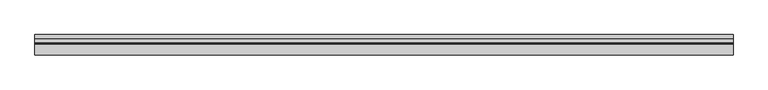
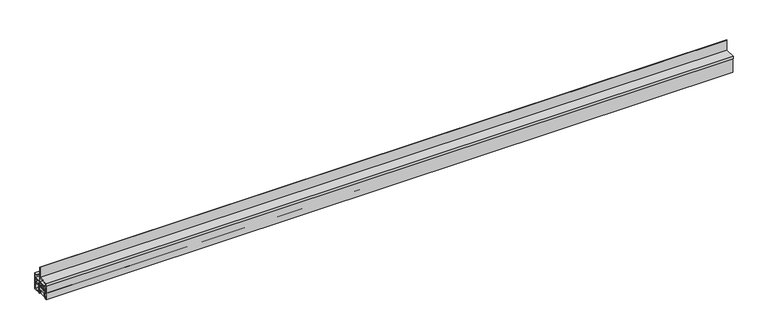
"""IFC4 building model written with IfcOpenShell, lengths in millimetres: proxy geometry, Window frame005 2183 : Window frame005 2183."""

from ifc_helpers import new_model, si_unit, frame, origin, place, context, project, spatial, polyline, outline, extrude, source, transform, mapped, element, save


def generic_models_6b3d6bd2(model_context):
    return source(origin(), model_context, "Body", "SweptSolid", [
        extrude(outline(polyline([(9726.5736227, 39484.9385304), (9727.747735, 39484.9385304), (9728.4102621, 39482.3483128), (9728.4102621, 39480.4869499), (9727.7746229, 39477.6249737), (9726.4212579, 39477.6249737), (9725.9975166, 39480.0838666), (9723.7713026, 39480.0838666), (9723.7713026, 39482.4968666), (9725.9982105, 39482.4968666), (9726.5736227, 39484.9385304)])), frame((3694.2883192, 0.0, 0.0), z_axis=(1.0, 0.0, 0.0), x_axis=(0.0, 1.0, 0.0)), (0.0, 0.0, 1.0), 2000.0),
        extrude(outline(polyline([(9755.7161826, 39477.6249737), (9754.5420703, 39477.6249737), (9753.8795432, 39480.2151913), (9753.8795432, 39482.0765542), (9754.5151824, 39484.9385304), (9755.8685473, 39484.9385304), (9756.2922886, 39482.4796375), (9758.5185026, 39482.4796375), (9758.5185026, 39480.0666375), (9756.2915948, 39480.0666375), (9755.7161826, 39477.6249737)])), frame((3694.2883192, 0.0, 0.0), z_axis=(1.0, 0.0, 0.0), x_axis=(0.0, 1.0, 0.0)), (0.0, 0.0, 1.0), 2000.0),
        extrude(outline(polyline([(3694.2883192, 9734.7568026), (3694.2883192, 9747.5330026), (5694.2883192, 9747.5330026), (5694.2883192, 9734.7568026), (3694.2883192, 9734.7568026)])), frame((0.0, 0.0, 39480.6381375), z_axis=(0.0, 0.0, 1.0), x_axis=(1.0, 0.0, 0.0)), (0.0, 0.0, 1.0), 9.525),
        extrude(outline(polyline([(9753.8576026, 39490.1631375), (9729.749919, 39490.1631375), (9727.984619, 39491.689029), (9727.984619, 39496.4603009), (9726.0827026, 39496.4603009), (9726.0827026, 39499.7389375), (9732.9007638, 39499.7389375), (9732.9007638, 39496.0415553), (9739.8141425, 39496.0415553), (9739.8141425, 39497.9101375), (9753.8576026, 39497.9101375), (9753.8576026, 39490.1631375)])), frame((3694.2883192, 0.0, 0.0), z_axis=(1.0, 0.0, 0.0), x_axis=(0.0, 1.0, 0.0)), (0.0, 0.0, 1.0), 2000.0),
        extrude(outline(polyline([(9778.8385026, 39477.4631375), (9756.2325026, 39477.4631375), (9756.2325026, 39479.6546368), (9757.5008807, 39479.6546368), (9757.5008807, 39478.7331375), (9758.7725026, 39478.7331375), (9758.7725026, 39483.8131375), (9757.5008807, 39483.8131375), (9757.5008807, 39482.9068417), (9756.2325026, 39482.9068417), (9756.2325026, 39485.0831375), (9758.7725026, 39485.0831375), (9758.7725026, 39497.9101375), (9736.1518446, 39497.9355375), (9736.1518446, 39499.3071375), (9760.1695026, 39499.3071375), (9760.1695026, 39478.8601375), (9777.4415026, 39478.8601375), (9777.4415026, 39493.5159375), (9774.0508822, 39493.5159375), (9774.0508822, 39498.5870442), (9775.3390149, 39498.5870442), (9776.4005173, 39496.9705166), (9775.4735631, 39494.9129375), (9778.8385026, 39494.9129375), (9778.8385026, 39477.4631375)])), frame((3694.2883192, 0.0, 0.0), z_axis=(1.0, 0.0, 0.0), x_axis=(0.0, 1.0, 0.0)), (0.0, 0.0, 1.0), 2000.0),
        extrude(outline(polyline([(9735.1468473, 39509.7841267), (9733.8805026, 39509.7841267), (9733.8805026, 39513.3533375), (9753.4385031, 39513.3533368), (9753.4385026, 39526.5558702), (9753.4385026, 39556.8834702), (9755.0133026, 39556.8834702), (9755.0133026, 39513.3533375), (9776.5525026, 39513.3533375), (9776.8065026, 39524.5039375), (9768.3483026, 39524.5039375), (9768.3483026, 39526.5359375), (9778.8385026, 39526.5359375), (9778.8385026, 39494.9129375), (9775.551216, 39494.9129375), (9776.8065026, 39497.4786952), (9776.8065026, 39499.7389375), (9736.1518446, 39499.7389375), (9736.1518446, 39497.9101375), (9739.0893772, 39497.9101375), (9739.0893772, 39496.5639375), (9734.6416892, 39496.5639375), (9734.6416892, 39499.7389375), (9733.1012905, 39499.7389375), (9733.1012905, 39501.7709375), (9737.6905026, 39501.7709375), (9737.6905026, 39511.3213375), (9735.1468473, 39511.3213375), (9735.1468473, 39509.7841267)]), holes=[polyline([(9767.4897498, 39510.1783375), (9767.4897498, 39511.3213375), (9759.2470473, 39511.3213375), (9759.2470473, 39510.1783375), (9752.6705617, 39510.1783375), (9752.6705617, 39511.3213375), (9743.6845244, 39511.3213375), (9743.6845244, 39510.1783375), (9739.7225026, 39510.1783375), (9739.7225026, 39506.5461375), (9739.7225026, 39502.9139375), (9747.2851294, 39502.9139375), (9747.2851294, 39501.7709375), (9754.0989026, 39501.7709375), (9754.0989026, 39502.9139375), (9759.2470473, 39502.9139375), (9759.2470473, 39501.7709375), (9762.8774031, 39501.7709375), (9762.8774031, 39502.9139375), (9772.8162468, 39502.9139375), (9772.8162468, 39501.7709375), (9776.2985026, 39501.7709375), (9776.2985026, 39506.5461375), (9776.2985026, 39511.3213375), (9772.8162468, 39511.3213375), (9772.8162468, 39510.1783375), (9767.4897498, 39510.1783375)])]), frame((3694.2883192, 0.0, 0.0), z_axis=(1.0, 0.0, 0.0), x_axis=(0.0, 1.0, 0.0)), (0.0, 0.0, 1.0), 2000.0),
        extrude(outline(polyline([(9720.6725026, 39520.1859375), (9720.6725026, 39527.5519375), (9752.4225026, 39527.5519375), (9752.4225026, 39558.2859375), (9753.4385026, 39558.2859375), (9753.4385026, 39526.5558702), (9721.6885026, 39526.5359375), (9721.6885026, 39520.1859375), (9720.6725026, 39520.1859375)])), frame((3694.2883192, 0.0, 0.0), z_axis=(1.0, 0.0, 0.0), x_axis=(0.0, 1.0, 0.0)), (0.0, 0.0, 1.0), 2000.0),
        extrude(outline(polyline([(9731.9247026, 39526.5359375), (9731.9247026, 39524.5039375), (9723.7205026, 39524.5039375), (9723.7205026, 39513.3533375), (9727.5305026, 39513.3533375), (9727.5305026, 39509.7841267), (9726.186283, 39509.7841267), (9726.186283, 39511.3213375), (9723.7205026, 39511.3213375), (9723.7205026, 39501.7709375), (9728.3097148, 39501.7709375), (9728.3097148, 39499.7389375), (9726.0827026, 39499.7389375), (9726.0827026, 39482.9550709), (9724.8127026, 39482.9550709), (9724.8127026, 39483.8131375), (9723.5427026, 39483.8131375), (9723.5427026, 39478.7331375), (9724.8127026, 39478.7331375), (9724.8127026, 39479.5925908), (9726.0827026, 39479.5925908), (9726.0827026, 39477.4631375), (9721.6885026, 39477.4631375), (9721.6885026, 39526.5359375), (9731.9247026, 39526.5359375)])), frame((3694.2883192, 0.0, 0.0), z_axis=(1.0, 0.0, 0.0), x_axis=(0.0, 1.0, 0.0)), (0.0, 0.0, 1.0), 2000.0),
    ])


if __name__ == "__main__":
    model = new_model("IFC4")
    model_context = context("Model", 3, world=origin())
    ifc_project = project(units=[si_unit("LENGTHUNIT", "METRE", prefix="MILLI")], contexts=[model_context])
    site = spatial("IfcSite", under=ifc_project)
    building = spatial("IfcBuilding", under=site)
    placement = place(None, origin())
    generic_models_shape = generic_models_6b3d6bd2(model_context)
    element("IfcBuildingElementProxy", 1, Name="Window frame005 2183 : Window frame005 2183", ObjectType="Window frame005 2183 : Window frame005 2183", at=placement, inside=building, context=model_context, shape_type="MappedRepresentation", body=[
        mapped(generic_models_shape, transform((0.0, 0.0, 0.0), x_axis=(1.0, 0.0, 0.0), y_axis=(0.0, 1.0, 0.0), z_axis=(0.0, 0.0, 1.0))),
    ])
    save(model, "model.ifc")

# Revit data of these elements
# Type "Window frame005 2183 : Window frame005 2183"
#   NameOverride = "Window frame005"
# Element 1 (IfcBuildingElementProxy, "Window frame005 2183 : Window frame005 2183")
#   Materials on its faces: "FLEETWOOD SERIES 250-T-04 FIXED UNIT WINDOW FRAME"
# Materials
#   "FLEETWOOD SERIES 250-T-04 FIXED UNIT WINDOW FRAME": class "Unassigned", colour RGB 128 128 128, transparency 0
